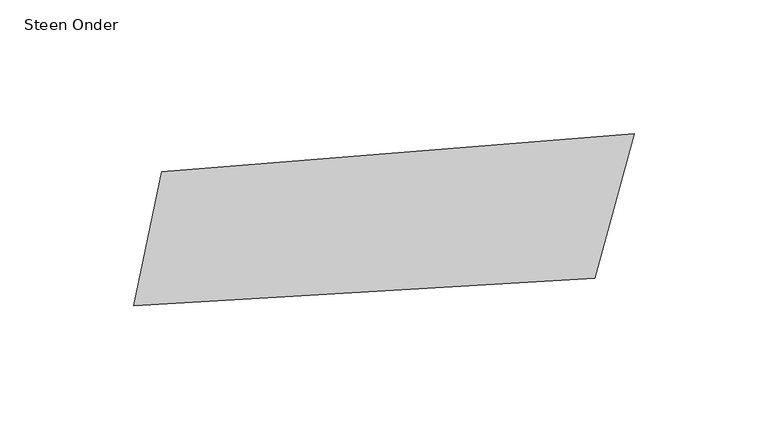
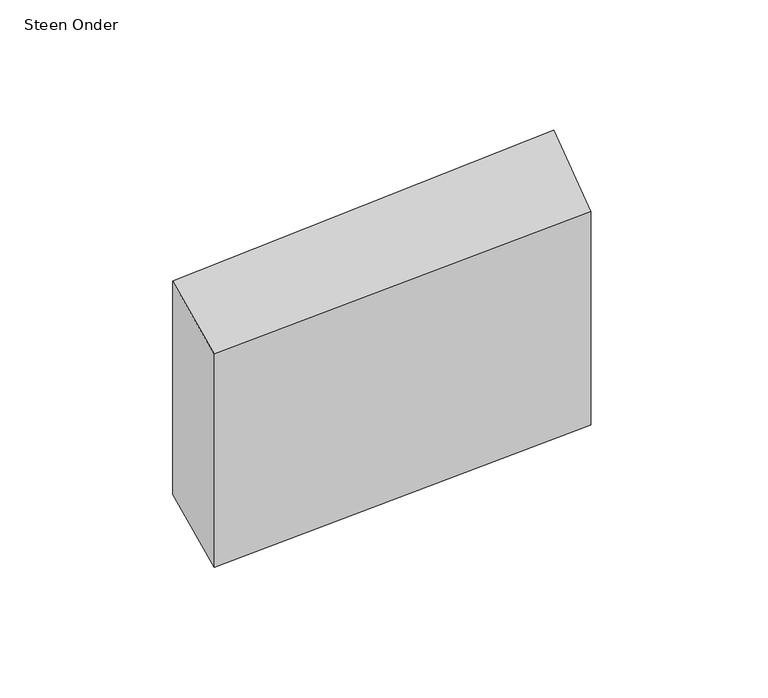
"""IFC4 building model written with IfcOpenShell, lengths in millimetres: proxy geometry, 00_GMA_steen_versie_4 : Steen Onder."""

from ifc_helpers import new_model, si_unit, frame, origin, place, context, project, spatial, polyline, outline, extrude, source, transform, mapped, element, save


def steen_onder_1977260d(model_context):
    return source(origin(), model_context, "Body", "SweptSolid", [
        extrude(outline(polyline([(190.3343827, 70.658415), (175.5684349, 16.5220185), (3.0255666, 6.1935349), (13.5454442, 56.3968082), (190.3343827, 70.658415)])), frame((0.0, 0.0, -100.0), z_axis=(0.0, 0.0, 1.0), x_axis=(1.0, 0.0, 0.0)), (0.0, 0.0, 1.0), 100.0),
    ])


if __name__ == "__main__":
    model = new_model("IFC4")
    model_context = context("Model", 3, world=origin())
    ifc_project = project(units=[si_unit("LENGTHUNIT", "METRE", prefix="MILLI")], contexts=[model_context])
    site = spatial("IfcSite", under=ifc_project)
    building = spatial("IfcBuilding", under=site)
    placement = place(None, origin())
    steen_onder_shape = steen_onder_1977260d(model_context)
    element("IfcBuildingElementProxy", 1, Name="00_GMA_steen_versie_4 : Steen Onder", ObjectType="00_GMA_steen_versie_4 : Steen Onder", at=placement, inside=building, context=model_context, shape_type="MappedRepresentation", body=[
        mapped(steen_onder_shape, transform((0.0, 0.0, 0.0), x_axis=(1.0, 0.0, 0.0), y_axis=(0.0, 1.0, 0.0), z_axis=(0.0, 0.0, 1.0))),
    ])
    save(model, "model.ifc")

# Revit data of these elements
# Type "00_GMA_steen_versie_4 : Steen Onder"
#   StootVoegHalfBoven [instance default] = 5 mm
#   StootVoegHalf [instance default] = 5 mm
#   StootVoegBreedteOnder = 10 mm
#   StootVoegBreedteBoven = 10 mm
#   Steendikte = 100 mm
#   LintVoegOnderHalf = 0 mm
#   LintVoegOnder = 0 mm
#   LintVoegBovenHalf = 5 mm
#   LintVoegBoven = 10 mm
#   materiaal = none
#   MateriaalVoeg = none
#   Default Elevation = 0
